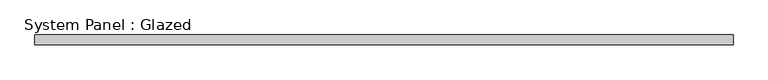
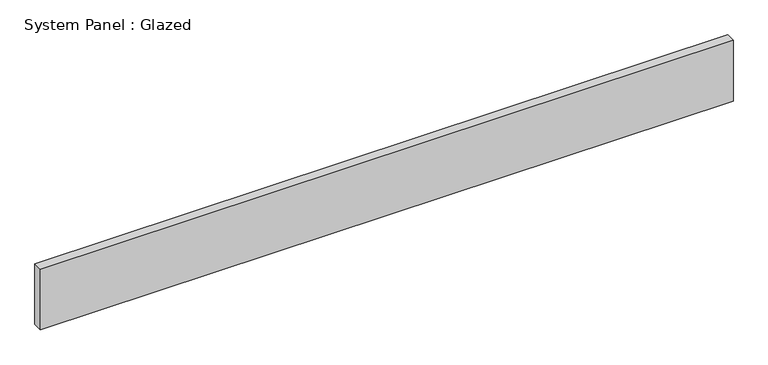
"""IFC4 building model written with IfcOpenShell, lengths in millimetres: plate geometry, System Panel : Glazed."""

from ifc_helpers import new_model, si_unit, origin, origin_with_axes, place, context, project, spatial, polyline, outline, extrude, source, transform, mapped, element, save


def system_panel_glazed_f4345ae3(model_context):
    return source(origin(), model_context, "Body", "SweptSolid", [
        extrude(outline(polyline([(914.4, -44.45), (-914.4, -44.45), (-914.4, -19.05), (914.4, -19.05), (914.4, -44.45)])), origin_with_axes(), (0.0, 0.0, 1.0), 169.2731269),
    ])


if __name__ == "__main__":
    model = new_model("IFC4")
    model_context = context("Model", 3, world=origin())
    ifc_project = project(units=[si_unit("LENGTHUNIT", "METRE", prefix="MILLI")], contexts=[model_context])
    site = spatial("IfcSite", under=ifc_project)
    building = spatial("IfcBuilding", under=site)
    placement = place(None, origin())
    system_panel_glazed_shape = system_panel_glazed_f4345ae3(model_context)
    element("IfcPlate", 1, ObjectType="System Panel : Glazed", at=placement, inside=building, context=model_context, shape_type="MappedRepresentation", body=[
        mapped(system_panel_glazed_shape, transform((0.0, 0.0, 0.0), x_axis=(1.0, 0.0, 0.0), y_axis=(0.0, 1.0, 0.0), z_axis=(0.0, 0.0, 1.0))),
    ])
    save(model, "model.ifc")

# Revit data of these elements
# Type "System Panel : Glazed"
#   Construction Type Id = "GSP4R"
#   Analytic Construction = "1/8 in Pilkington single glazing"
#   Visual Light Transmittance = 0.9
#   Solar Heat Gain Coefficient = 0.86
#   Heat Transfer Coefficient (U) = 1.18115 BTU/(h·ft²·°F)
#   Define Thermal Properties by = 1
# Element 1 (IfcPlate, "System Panel : Glazed")
#   Materials on its faces: "Glass"
# Materials
#   "Glass": class "Glass", colour RGB 0 128 192, transparency 0.75, Description = "Soda Lime Glass", Cost = 0
